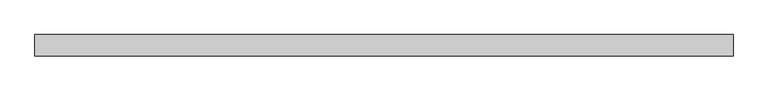
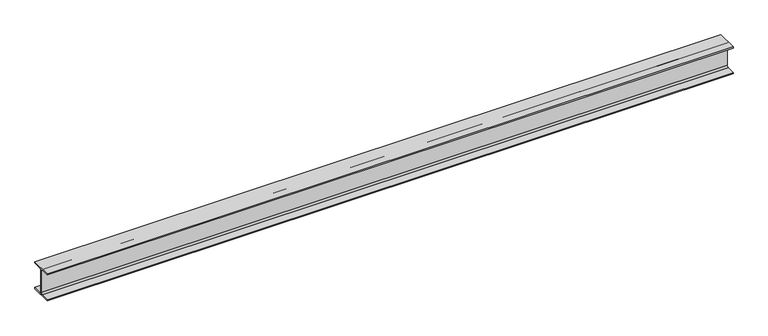
"""IFC4 building model written with IfcOpenShell, lengths in millimetres: beam geometry, 0912_Steel Framing_H-KSD3502 : H_SB_ASB_H-340x250x9x14."""

from ifc_helpers import new_model, si_unit, point, frame, frame_2d, origin, place, context, project, spatial, polyline, circle_curve, trimmed, segment, composite_curve, outline, extrude, source, transform, mapped, element, save


def beam_b521a539(model_context):
    return source(origin(), model_context, "Body", "SweptSolid", [
        extrude(outline(composite_curve([segment(polyline([(125.0, -156.0), (125.0, -170.0), (-125.0, -170.0), (-125.0, -156.0), (-24.5, -156.0)]), True, "CONTINUOUS"), segment(trimmed(circle_curve(frame_2d((-24.5, -136.0)), 20.0), [point((-24.5, -156.0))], [point((-4.5, -136.0))], True, "CARTESIAN"), True, "CONTINUOUS"), segment(polyline([(-4.5, -136.0), (-4.5, 136.0)]), True, "CONTINUOUS"), segment(trimmed(circle_curve(frame_2d((-24.5, 136.0)), 20.0), [point((-4.5, 136.0))], [point((-24.5, 156.0))], True, "CARTESIAN"), True, "CONTINUOUS"), segment(polyline([(-24.5, 156.0), (-125.0, 156.0), (-125.0, 170.0), (125.0, 170.0), (125.0, 156.0), (24.5, 156.0)]), True, "CONTINUOUS"), segment(trimmed(circle_curve(frame_2d((24.5, 136.0)), 20.0), [point((24.5, 156.0))], [point((4.5, 136.0))], True, "CARTESIAN"), True, "CONTINUOUS"), segment(polyline([(4.5, 136.0), (4.5, -136.0)]), True, "CONTINUOUS"), segment(trimmed(circle_curve(frame_2d((24.5, -136.0)), 20.0), [point((4.5, -136.0))], [point((24.5, -156.0))], True, "CARTESIAN"), True, "CONTINUOUS"), segment(polyline([(24.5, -156.0), (125.0, -156.0)]), True, "CONTINUOUS")], self_intersect=False)), frame((-4087.3, 0.0, 0.0), z_axis=(1.0, 0.0, 0.0), x_axis=(0.0, 1.0, 0.0)), (0.0, 0.0, 1.0), 8174.6),
    ])


if __name__ == "__main__":
    model = new_model("IFC4")
    model_context = context("Model", 3, world=origin())
    ifc_project = project(units=[si_unit("LENGTHUNIT", "METRE", prefix="MILLI")], contexts=[model_context])
    site = spatial("IfcSite", under=ifc_project)
    building = spatial("IfcBuilding", under=site)
    placement = place(None, origin())
    beam_shape = beam_b521a539(model_context)
    element("IfcBeam", 1, ObjectType="0912_Steel Framing_H-KSD3502 : H_SB_ASB_H-340x250x9x14", at=placement, inside=building, context=model_context, shape_type="MappedRepresentation", body=[
        mapped(beam_shape, transform((0.0, 0.0, 0.0), x_axis=(1.0, 0.0, 0.0), y_axis=(0.0, 1.0, 0.0), z_axis=(0.0, 0.0, 1.0))),
    ])
    save(model, "model.ifc")

# Revit data of these elements
# Type "0912_Steel Framing_H-KSD3502 : H_SB_ASB_H-340x250x9x14"
#   H_WM Code_1 = "S01AA002-00001 | Main Steel Structure Fabrication Work | Shelter/Building | Medium Steel - Standard (90KG/M>Weight≥30KG/M) | Material: (   )"
#   H_WM Code_2 = "S03AA028-00001 | Main Steel Structure Erection Work | Shelter/Building | Medium Steel (90KG/M>Weight≥30KG/M) | Material: (   )"
#   H_WM Code_3 = "S01AA010-00001 | Main Steel Structure Fabrication Work | Shelter/Building | Steel Painting/Coating | for Non-Fireproofed Steel Surface, Surface Preparation, Primer, Second & Final Coat | Material: (   )"
#   H_Q'ty Cal Type Tag = "SB-Q2"
#   Width = 25.0 cm
#   Web Thickness = 0.9 cm
#   Web Fillet = 2.0 cm
#   Warping Constant = 969000.0 cm⁶
#   W = 0
#   Torsional Moment of Inertia = 53.6551 cm⁴
#   Section Area = 101.5 cm²
#   Plastic Modulus weak axis = 447.0 cm³
#   Plastic Modulus strong axis = 1410.0 cm³
#   Perimeter = 1.63 m²/m
#   Nominal Weight = 79.70 kgf/m
#   Moment of Inertia weak axis = 3650.00 cm⁴
#   Moment of Inertia strong axis = 21700.00 cm⁴
#   Height = 34.0 cm
#   Flange Thickness = 1.4 cm
#   Elastic Modulus weak axis = 292.0 cm³
#   Elastic Modulus strong axis = 1280.0 cm³
#   Centroid Vertical = 17.0 cm
#   Centroid Horizontal = 12.5 cm
#   Ix = 217000000
#   Length [instance default] = 1.5240 m
#   Zx = 1410000
#   b = 0.2500 m
#   h = 0.3400 m
#   r = 0.0200 m
#   s = 0.0090 m
#   t = 0.0140 m
#   A = 0.01015 m²
#   Structural Material [instance default] = Steel, 45-345
#   Assembly Code = ""
# Element 1 (IfcBeam, "0912_Steel Framing_H-KSD3502 : H_SB_ASB_H-340x250x9x14")
#   Structural Material = none
# Materials
#   "Steel, 45-345": class "Metal", colour RGB 189 187 185, transparency 0, Description = "Steel 345 MPa", Cost = 0
